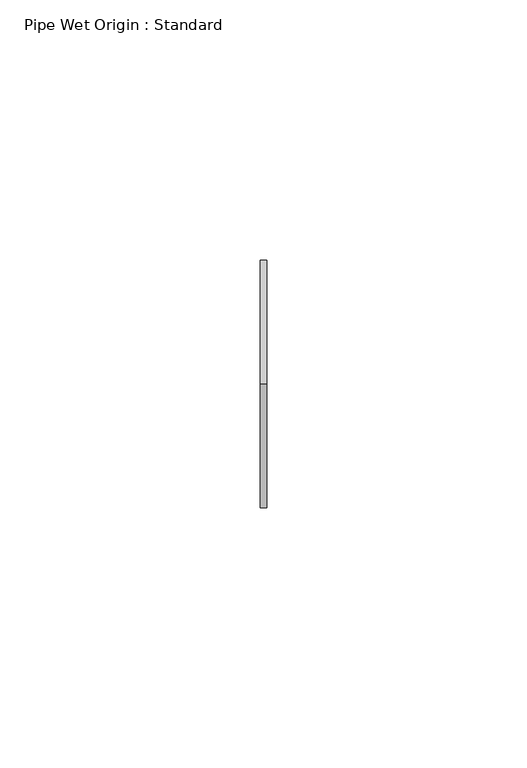
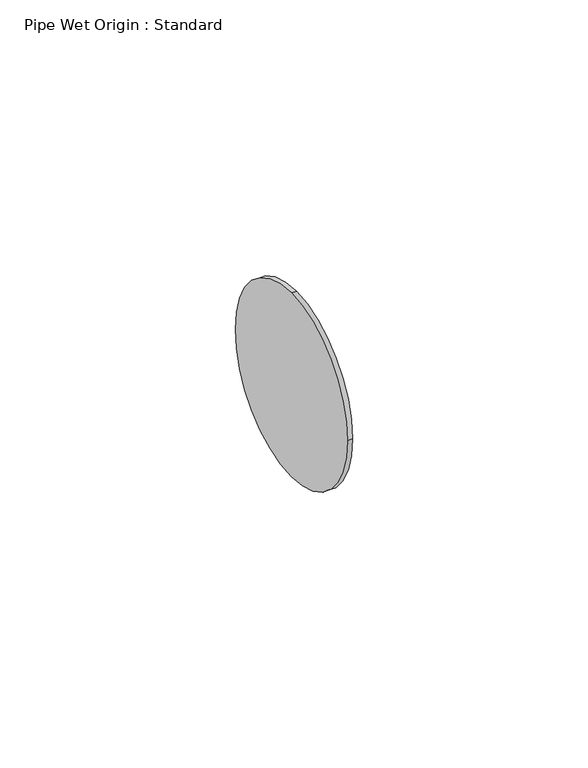
"""IFC4 building model written with IfcOpenShell, lengths in millimetres: proxy geometry, Pipe Wet Origin : Standard."""

import ifcopenshell
import ifcopenshell.guid

model = None  # the IFC model being written
_history = None  # IfcOwnerHistory: only IFC2X3 demands one
_inside = {}  # id of a spatial element -> (the spatial element, [elements in it])
_under = {}  # id of a project, library or spatial element -> (it, [spatial elements below it])
_declared = {}  # id of a project -> (the project, [libraries it declares])
_typed = {}  # id of a type object -> (the type object, [elements of that type])
_made_of = {}  # id of a material, layer set ... -> (it, [elements and type objects made of it])


def new_model(schema):
    """Start an empty IFC model of exactly this schema.

    Asked for "IFC4X3", IfcOpenShell would pick the latest addendum, in which some entities
    have other attributes; the version numbers below select the first issue.
    IFC2X3 requires an IfcOwnerHistory on every rooted entity: one is made here for all.
    """
    global model, _history
    if schema == "IFC4X3":
        model = ifcopenshell.file(schema_version=(4, 3, 0, 0))
    else:
        model = ifcopenshell.file(schema=schema)
    _inside.clear()
    _under.clear()
    _declared.clear()
    _typed.clear()
    _made_of.clear()
    _history = None
    if model.schema == "IFC2X3":
        org = make("IfcOrganization", Name="unknown")
        user = make(
            "IfcPersonAndOrganization",
            ThePerson=make("IfcPerson", FamilyName="unknown"),
            TheOrganization=org,
        )
        app = make(
            "IfcApplication",
            ApplicationDeveloper=org,
            Version="unknown",
            ApplicationFullName="unknown",
            ApplicationIdentifier="unknown",
        )
        _history = make(
            "IfcOwnerHistory",
            OwningUser=user,
            OwningApplication=app,
            ChangeAction="ADDED",
            CreationDate=0,
        )
    return model


def make(cls, **values):
    """One entity of the class cls with the attributes given. An attribute that is None is left unset."""
    return model.create_entity(
        cls, **{name: value for name, value in values.items() if value is not None}
    )


def rooted(cls, **values):
    """An entity with a GlobalId (a new one), such as an element, a storey or a relation."""
    return make(cls, GlobalId=ifcopenshell.guid.new(), OwnerHistory=_history, **values)


def si_unit(unit_type, name, prefix=None):
    """IfcSIUnit, for example si_unit("LENGTHUNIT", "METRE", prefix="MILLI")."""
    return make("IfcSIUnit", UnitType=unit_type, Prefix=prefix, Name=name)


def assignment(units):
    """IfcUnitAssignment: the units of a project."""
    return None if units is None else make("IfcUnitAssignment", Units=units)


def point(xyz):
    """IfcCartesianPoint."""
    return None if xyz is None else make("IfcCartesianPoint", Coordinates=xyz)


def direction(xyz):
    """IfcDirection."""
    return None if xyz is None else make("IfcDirection", DirectionRatios=xyz)


def frame(location, z_axis=None, x_axis=None):
    """IfcAxis2Placement3D, a coordinate frame: its origin and axes. An axis left out is left unset."""
    return make(
        "IfcAxis2Placement3D",
        Location=point(location),
        Axis=direction(z_axis),
        RefDirection=direction(x_axis),
    )


def frame_2d(location, x_axis=None):
    """IfcAxis2Placement2D, a coordinate frame in the plane: its origin and x axis."""
    return make(
        "IfcAxis2Placement2D", Location=point(location), RefDirection=direction(x_axis)
    )


def origin():
    """The frame at (0, 0, 0) with its axes left unset."""
    return frame((0.0, 0.0, 0.0))


def origin_2d():
    """The frame at (0, 0) in the plane with its x axis left unset."""
    return frame_2d((0.0, 0.0))


def place(relative_to, where):
    """IfcLocalPlacement: puts the frame where relative to a parent placement (None: the world)."""
    return make(
        "IfcLocalPlacement", PlacementRelTo=relative_to, RelativePlacement=where
    )


def context(
    kind, dimensions, precision=None, world=None, true_north=None, identifier=None
):
    """IfcGeometricRepresentationContext, for example the 3D "Model" context."""
    return make(
        "IfcGeometricRepresentationContext",
        ContextIdentifier=identifier,
        ContextType=kind,
        CoordinateSpaceDimension=dimensions,
        Precision=precision,
        WorldCoordinateSystem=world,
        TrueNorth=true_north,
    )


def project(units=None, contexts=None):
    """IfcProject with its units and contexts."""
    return rooted(
        "IfcProject",
        Name="project",
        RepresentationContexts=contexts,
        UnitsInContext=assignment(units),
    )


def spatial(cls, under=None, at=None, **own):
    """A site, building, storey or space (cls), placed at a placement, below another one or the project."""
    s = rooted(cls, ObjectPlacement=at, **own)
    if under is not None:
        _under.setdefault(under.id(), (under, []))[1].append(s)
    return s


def circle_curve(where, radius):
    """IfcCircle in the frame where."""
    return make("IfcCircle", Position=where, Radius=radius)


def trimmed(basis, trim1, trim2, sense, master):
    """IfcTrimmedCurve: the piece of a basis curve between two trims."""
    return make(
        "IfcTrimmedCurve",
        BasisCurve=basis,
        Trim1=trim1,
        Trim2=trim2,
        SenseAgreement=sense,
        MasterRepresentation=master,
    )


def segment(curve, same_sense, transition):
    """IfcCompositeCurveSegment."""
    return make(
        "IfcCompositeCurveSegment",
        Transition=transition,
        SameSense=same_sense,
        ParentCurve=curve,
    )


def composite_curve(segments, self_intersect=None):
    """IfcCompositeCurve: segments joined end to end."""
    return make("IfcCompositeCurve", Segments=segments, SelfIntersect=self_intersect)


def outline(outer, holes=None, kind="AREA"):
    """IfcArbitraryClosedProfileDef: a profile drawn as a closed curve; with holes, ...WithVoids."""
    if holes is None:
        return make("IfcArbitraryClosedProfileDef", ProfileType=kind, OuterCurve=outer)
    return make(
        "IfcArbitraryProfileDefWithVoids",
        ProfileType=kind,
        OuterCurve=outer,
        InnerCurves=holes,
    )


def extrude(swept, where, along, depth):
    """IfcExtrudedAreaSolid: the profile swept, set in the frame where, extruded along a direction by depth."""
    return make(
        "IfcExtrudedAreaSolid",
        SweptArea=swept,
        Position=where,
        ExtrudedDirection=direction(along),
        Depth=depth,
    )


def shape(context_of_items, identifier, shape_type, items):
    """IfcShapeRepresentation: the items that make up one representation, for example the "Body"."""
    return make(
        "IfcShapeRepresentation",
        ContextOfItems=context_of_items,
        RepresentationIdentifier=identifier,
        RepresentationType=shape_type,
        Items=items,
    )


def source(mapping_origin, context_of_items, identifier, shape_type, items):
    """IfcRepresentationMap: a shape defined once, which mapped items show again and again."""
    return make(
        "IfcRepresentationMap",
        MappingOrigin=mapping_origin,
        MappedRepresentation=shape(context_of_items, identifier, shape_type, items),
    )


def transform(
    local_origin,
    x_axis=None,
    y_axis=None,
    z_axis=None,
    scale=None,
    scale2=None,
    scale3=None,
    uniform=True,
):
    """IfcCartesianTransformationOperator3D, or its non-uniform kind. x_axis, y_axis, z_axis: its Axis1, 2, 3."""
    if uniform:
        return make(
            "IfcCartesianTransformationOperator3D",
            Axis1=direction(x_axis),
            Axis2=direction(y_axis),
            LocalOrigin=point(local_origin),
            Scale=scale,
            Axis3=direction(z_axis),
        )
    return make(
        "IfcCartesianTransformationOperator3DnonUniform",
        Axis1=direction(x_axis),
        Axis2=direction(y_axis),
        LocalOrigin=point(local_origin),
        Scale=scale,
        Axis3=direction(z_axis),
        Scale2=scale2,
        Scale3=scale3,
    )


def mapped(mapping_source, mapping_target):
    """IfcMappedItem: shows the shape of a source again, moved by a transform."""
    return make(
        "IfcMappedItem", MappingSource=mapping_source, MappingTarget=mapping_target
    )


def made_of(thing, what):
    """Note that an element or type object is made of a material, layer set ...; save() writes the relation."""
    if what is not None:
        _made_of.setdefault(what.id(), (what, []))[1].append(thing)
    return thing


def element(
    cls,
    number,
    at=None,
    inside=None,
    cuts=None,
    type_object=None,
    material=None,
    context=None,
    identifier="Body",
    shape_type=None,
    held_by="IfcProductDefinitionShape",
    body=None,
    shapes=None,
    **own,
):
    """One element of the class cls, such as IfcWall. Its Tag is "e" and its number.

    at: its placement. inside: the storey or other place that contains it. cuts: it is an
    opening in that element (IfcRelVoidsElement). A single representation is given by context,
    identifier, shape_type and body (its items); several are given by shapes. held_by: the class
    of the entity that holds the representations. save() writes the other relations.
    """
    e = rooted(cls, Tag="e%d" % number, ObjectPlacement=at, **own)
    if body is not None:
        shapes = [shape(context, identifier, shape_type, body)]
    if shapes is not None:
        e.Representation = make(held_by, Representations=shapes)
    if inside is not None:
        _inside.setdefault(inside.id(), (inside, []))[1].append(e)
    if cuts is not None:
        rooted(
            "IfcRelVoidsElement", RelatingBuildingElement=cuts, RelatedOpeningElement=e
        )
    if type_object is not None:
        _typed.setdefault(type_object.id(), (type_object, []))[1].append(e)
    return made_of(e, material)


def aggregate(whole, parts):
    """IfcRelAggregates: a whole, such as a stair, and the parts it consists of."""
    return rooted("IfcRelAggregates", RelatingObject=whole, RelatedObjects=parts)


def save(model, path):
    """Write the relations noted so far, then the file.

    IfcRelAggregates (storeys below a building ...), IfcRelContainedInSpatialStructure (elements
    in a storey), IfcRelDefinesByType, IfcRelAssociatesMaterial and IfcRelDeclares: one each for
    every whole, place, type object, material and project.
    """
    for whole, parts in _under.values():
        aggregate(whole, parts)
    for where, things in _inside.values():
        rooted(
            "IfcRelContainedInSpatialStructure",
            RelatedElements=things,
            RelatingStructure=where,
        )
    for kind, things in _typed.values():
        rooted("IfcRelDefinesByType", RelatedObjects=things, RelatingType=kind)
    for what, things in _made_of.values():
        rooted("IfcRelAssociatesMaterial", RelatedObjects=things, RelatingMaterial=what)
    for by, libraries in _declared.values():
        rooted("IfcRelDeclares", RelatingContext=by, RelatedDefinitions=libraries)
    model.write(path)


def pipe_wet_origin_standard_146eebac(model_context):
    return source(origin(), model_context, "Body", "SweptSolid", [
        extrude(outline(composite_curve([segment(trimmed(circle_curve(origin_2d(), 23.8125), [point((0.0, 23.8125))], [point((23.8125, 0.0))], False, "CARTESIAN"), True, "CONTINUOUS"), segment(trimmed(circle_curve(origin_2d(), 23.8125), [point((23.8125, 0.0))], [point((0.0, -23.8125))], False, "CARTESIAN"), True, "CONTINUOUS"), segment(trimmed(circle_curve(origin_2d(), 23.8125), [point((0.0, -23.8125))], [point((-23.8125, 0.0))], False, "CARTESIAN"), True, "CONTINUOUS"), segment(trimmed(circle_curve(origin_2d(), 23.8125), [point((-23.8125, 0.0))], [point((0.0, 23.8125))], False, "CARTESIAN"), True, "CONTINUOUS")], self_intersect=False)), frame((0.0, 0.0, 0.0), z_axis=(1.0, 0.0, 0.0), x_axis=(0.0, 1.0, 0.0)), (0.0, 0.0, 1.0), 1.27),
        extrude(outline(composite_curve([segment(trimmed(circle_curve(origin_2d(), 23.8125), [point((0.0, 23.8125))], [point((23.8125, 0.0))], False, "CARTESIAN"), True, "CONTINUOUS"), segment(trimmed(circle_curve(origin_2d(), 23.8125), [point((23.8125, 0.0))], [point((0.0, -23.8125))], False, "CARTESIAN"), True, "CONTINUOUS"), segment(trimmed(circle_curve(origin_2d(), 23.8125), [point((0.0, -23.8125))], [point((-23.8125, 0.0))], False, "CARTESIAN"), True, "CONTINUOUS"), segment(trimmed(circle_curve(origin_2d(), 23.8125), [point((-23.8125, 0.0))], [point((0.0, 23.8125))], False, "CARTESIAN"), True, "CONTINUOUS")], self_intersect=False)), frame((0.0, 0.0, 0.0), z_axis=(1.0, 0.0, 0.0), x_axis=(0.0, 1.0, 0.0)), (0.0, 0.0, 1.0), 1.27),
    ])


if __name__ == "__main__":
    model = new_model("IFC4")
    model_context = context("Model", 3, world=origin())
    ifc_project = project(units=[si_unit("LENGTHUNIT", "METRE", prefix="MILLI")], contexts=[model_context])
    site = spatial("IfcSite", under=ifc_project)
    building = spatial("IfcBuilding", under=site)
    placement = place(None, origin())
    pipe_wet_origin_standard_shape = pipe_wet_origin_standard_146eebac(model_context)
    element("IfcBuildingElementProxy", 1, Name="Pipe Wet Origin : Standard", ObjectType="Pipe Wet Origin : Standard", at=placement, inside=building, context=model_context, shape_type="MappedRepresentation", body=[
        mapped(pipe_wet_origin_standard_shape, transform((0.0, 0.0, 0.0), x_axis=(1.0, 0.0, 0.0), y_axis=(0.0, 1.0, 0.0), z_axis=(0.0, 0.0, 1.0))),
    ])
    save(model, "model.ifc")

# Revit data of these elements
# Type "Pipe Wet Origin : Standard"
#   Lookup Table Name [instance default] = "Pipe Fitting Sizes"
#   WaterFlow [instance default] = 0 GPM
#   Radius [instance default] = 2 3/16"
#   Nominal Size [instance default] = 4"
#   Nominal Radius [instance default] = 2"
#   Insulation Thickness [instance default] = 0"
#   Insulation Radius [instance default] = 2 3/16"
#   IsCustom [instance default] = no
#   Assembly Code = ""
# Element 1 (IfcBuildingElementProxy, "Pipe Wet Origin : Standard")
#   Radius = 15/16"
#   Nominal Size = 1 1/2"
#   Nominal Radius = 3/4"
#   Insulation Radius = 15/16"
